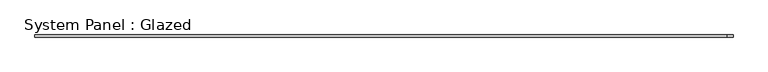
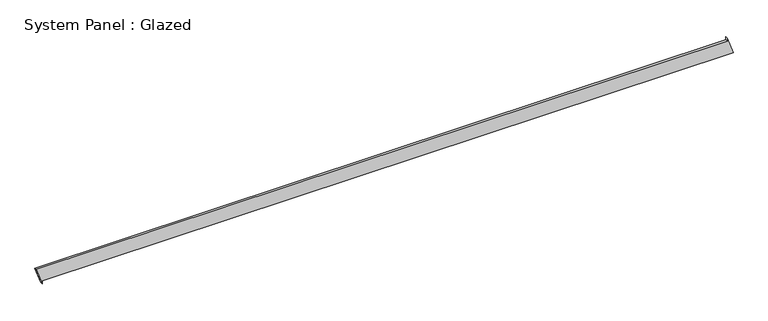
"""IFC4 building model written with IfcOpenShell, lengths in millimetres: plate geometry, System Panel : Glazed."""

from ifc_helpers import new_model, si_unit, frame, origin, place, context, project, spatial, polyline, outline, extrude, source, transform, mapped, element, save


def system_panel_glazed_a3f05b8f(model_context):
    return source(origin(), model_context, "Body", "SweptSolid", [
        extrude(outline(polyline([(0.0, -3958.100606), (35.3553391, -3958.100606), (35.3553391, 4027.4732247), (235.6210783, 3958.4712631), (200.2657393, 3958.4719436), (200.1120339, -4027.4732247), (0.0, -3958.100606)])), frame((0.0, -49.5, 0.0), z_axis=(0.0, 1.0, 0.0), x_axis=(0.0, 0.0, 1.0)), (0.0, 0.0, 1.0), 25.0),
    ])


if __name__ == "__main__":
    model = new_model("IFC4")
    model_context = context("Model", 3, world=origin())
    ifc_project = project(units=[si_unit("LENGTHUNIT", "METRE", prefix="MILLI")], contexts=[model_context])
    site = spatial("IfcSite", under=ifc_project)
    building = spatial("IfcBuilding", under=site)
    placement = place(None, origin())
    system_panel_glazed_shape = system_panel_glazed_a3f05b8f(model_context)
    element("IfcPlate", 1, ObjectType="System Panel : Glazed", at=placement, inside=building, context=model_context, shape_type="MappedRepresentation", body=[
        mapped(system_panel_glazed_shape, transform((0.0, 0.0, 0.0), x_axis=(1.0, 0.0, 0.0), y_axis=(0.0, 1.0, 0.0), z_axis=(0.0, 0.0, 1.0))),
    ])
    save(model, "model.ifc")

# Revit data of these elements
# Element 1 (IfcPlate, "System Panel : Glazed")
#   Materials on its faces: "Glass"
# Materials
#   "Glass": class "Glass", colour RGB 218 227 224, transparency 0.85, Description = "Soda Lime Glass", Cost = 0
